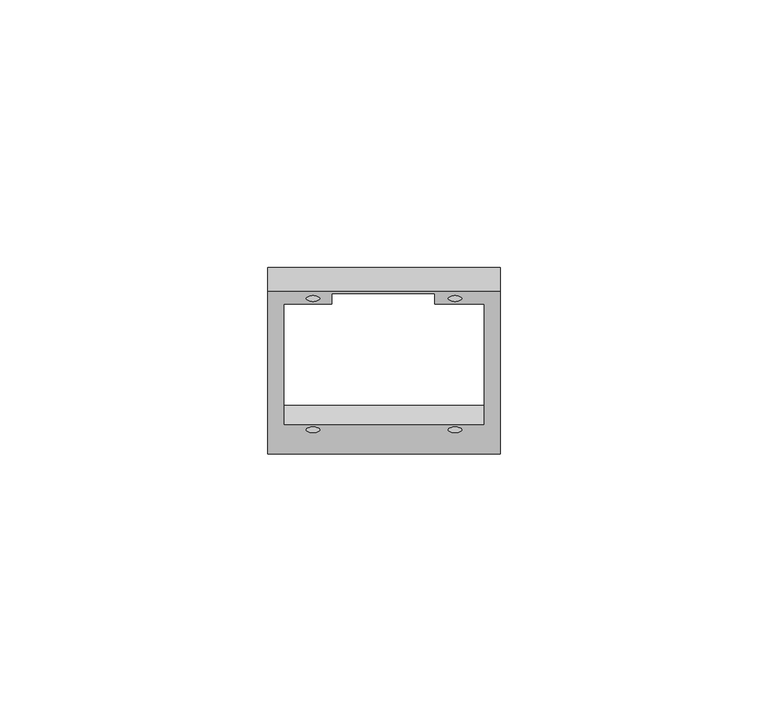
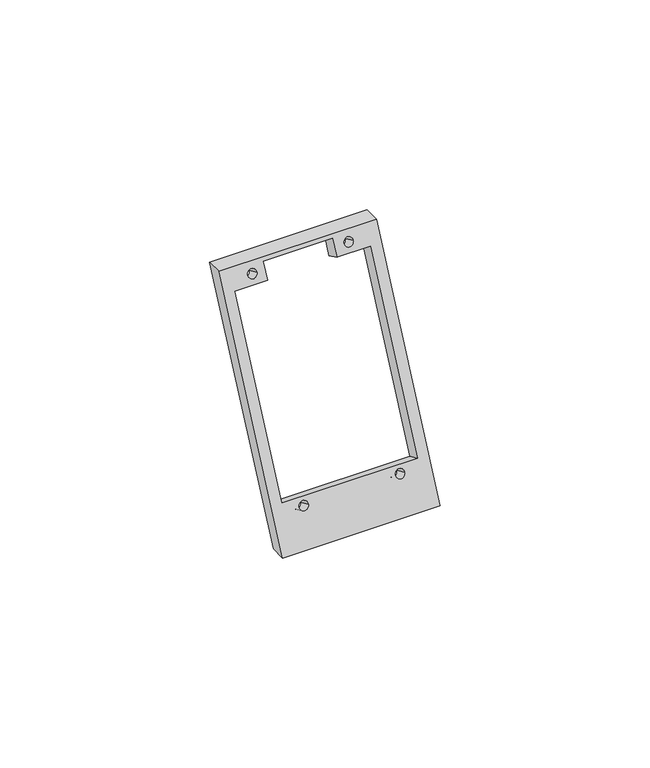
"""IFC4 building model written with IfcOpenShell, lengths in millimetres: furniture geometry, MOLDURA TELA : MOLDURA TELA."""

import ifcopenshell
import ifcopenshell.guid

model = None  # the IFC model being written
_history = None  # IfcOwnerHistory: only IFC2X3 demands one
_inside = {}  # id of a spatial element -> (the spatial element, [elements in it])
_under = {}  # id of a project, library or spatial element -> (it, [spatial elements below it])
_declared = {}  # id of a project -> (the project, [libraries it declares])
_typed = {}  # id of a type object -> (the type object, [elements of that type])
_made_of = {}  # id of a material, layer set ... -> (it, [elements and type objects made of it])


def new_model(schema):
    """Start an empty IFC model of exactly this schema.

    Asked for "IFC4X3", IfcOpenShell would pick the latest addendum, in which some entities
    have other attributes; the version numbers below select the first issue.
    IFC2X3 requires an IfcOwnerHistory on every rooted entity: one is made here for all.
    """
    global model, _history
    if schema == "IFC4X3":
        model = ifcopenshell.file(schema_version=(4, 3, 0, 0))
    else:
        model = ifcopenshell.file(schema=schema)
    _inside.clear()
    _under.clear()
    _declared.clear()
    _typed.clear()
    _made_of.clear()
    _history = None
    if model.schema == "IFC2X3":
        org = make("IfcOrganization", Name="unknown")
        user = make(
            "IfcPersonAndOrganization",
            ThePerson=make("IfcPerson", FamilyName="unknown"),
            TheOrganization=org,
        )
        app = make(
            "IfcApplication",
            ApplicationDeveloper=org,
            Version="unknown",
            ApplicationFullName="unknown",
            ApplicationIdentifier="unknown",
        )
        _history = make(
            "IfcOwnerHistory",
            OwningUser=user,
            OwningApplication=app,
            ChangeAction="ADDED",
            CreationDate=0,
        )
    return model


def make(cls, **values):
    """One entity of the class cls with the attributes given. An attribute that is None is left unset."""
    return model.create_entity(
        cls, **{name: value for name, value in values.items() if value is not None}
    )


def rooted(cls, **values):
    """An entity with a GlobalId (a new one), such as an element, a storey or a relation."""
    return make(cls, GlobalId=ifcopenshell.guid.new(), OwnerHistory=_history, **values)


def si_unit(unit_type, name, prefix=None):
    """IfcSIUnit, for example si_unit("LENGTHUNIT", "METRE", prefix="MILLI")."""
    return make("IfcSIUnit", UnitType=unit_type, Prefix=prefix, Name=name)


def assignment(units):
    """IfcUnitAssignment: the units of a project."""
    return None if units is None else make("IfcUnitAssignment", Units=units)


def point(xyz):
    """IfcCartesianPoint."""
    return None if xyz is None else make("IfcCartesianPoint", Coordinates=xyz)


def direction(xyz):
    """IfcDirection."""
    return None if xyz is None else make("IfcDirection", DirectionRatios=xyz)


def frame(location, z_axis=None, x_axis=None):
    """IfcAxis2Placement3D, a coordinate frame: its origin and axes. An axis left out is left unset."""
    return make(
        "IfcAxis2Placement3D",
        Location=point(location),
        Axis=direction(z_axis),
        RefDirection=direction(x_axis),
    )


def origin():
    """The frame at (0, 0, 0) with its axes left unset."""
    return frame((0.0, 0.0, 0.0))


def place(relative_to, where):
    """IfcLocalPlacement: puts the frame where relative to a parent placement (None: the world)."""
    return make(
        "IfcLocalPlacement", PlacementRelTo=relative_to, RelativePlacement=where
    )


def context(
    kind, dimensions, precision=None, world=None, true_north=None, identifier=None
):
    """IfcGeometricRepresentationContext, for example the 3D "Model" context."""
    return make(
        "IfcGeometricRepresentationContext",
        ContextIdentifier=identifier,
        ContextType=kind,
        CoordinateSpaceDimension=dimensions,
        Precision=precision,
        WorldCoordinateSystem=world,
        TrueNorth=true_north,
    )


def project(units=None, contexts=None):
    """IfcProject with its units and contexts."""
    return rooted(
        "IfcProject",
        Name="project",
        RepresentationContexts=contexts,
        UnitsInContext=assignment(units),
    )


def spatial(cls, under=None, at=None, **own):
    """A site, building, storey or space (cls), placed at a placement, below another one or the project."""
    s = rooted(cls, ObjectPlacement=at, **own)
    if under is not None:
        _under.setdefault(under.id(), (under, []))[1].append(s)
    return s


def polyline(points):
    """IfcPolyline through the points."""
    return make("IfcPolyline", Points=[point(p) for p in points])


def circle_curve(where, radius):
    """IfcCircle in the frame where."""
    return make("IfcCircle", Position=where, Radius=radius)


def shape(context_of_items, identifier, shape_type, items):
    """IfcShapeRepresentation: the items that make up one representation, for example the "Body"."""
    return make(
        "IfcShapeRepresentation",
        ContextOfItems=context_of_items,
        RepresentationIdentifier=identifier,
        RepresentationType=shape_type,
        Items=items,
    )


def source(mapping_origin, context_of_items, identifier, shape_type, items):
    """IfcRepresentationMap: a shape defined once, which mapped items show again and again."""
    return make(
        "IfcRepresentationMap",
        MappingOrigin=mapping_origin,
        MappedRepresentation=shape(context_of_items, identifier, shape_type, items),
    )


def transform(
    local_origin,
    x_axis=None,
    y_axis=None,
    z_axis=None,
    scale=None,
    scale2=None,
    scale3=None,
    uniform=True,
):
    """IfcCartesianTransformationOperator3D, or its non-uniform kind. x_axis, y_axis, z_axis: its Axis1, 2, 3."""
    if uniform:
        return make(
            "IfcCartesianTransformationOperator3D",
            Axis1=direction(x_axis),
            Axis2=direction(y_axis),
            LocalOrigin=point(local_origin),
            Scale=scale,
            Axis3=direction(z_axis),
        )
    return make(
        "IfcCartesianTransformationOperator3DnonUniform",
        Axis1=direction(x_axis),
        Axis2=direction(y_axis),
        LocalOrigin=point(local_origin),
        Scale=scale,
        Axis3=direction(z_axis),
        Scale2=scale2,
        Scale3=scale3,
    )


def mapped(mapping_source, mapping_target):
    """IfcMappedItem: shows the shape of a source again, moved by a transform."""
    return make(
        "IfcMappedItem", MappingSource=mapping_source, MappingTarget=mapping_target
    )


def made_of(thing, what):
    """Note that an element or type object is made of a material, layer set ...; save() writes the relation."""
    if what is not None:
        _made_of.setdefault(what.id(), (what, []))[1].append(thing)
    return thing


def element(
    cls,
    number,
    at=None,
    inside=None,
    cuts=None,
    type_object=None,
    material=None,
    context=None,
    identifier="Body",
    shape_type=None,
    held_by="IfcProductDefinitionShape",
    body=None,
    shapes=None,
    **own,
):
    """One element of the class cls, such as IfcWall. Its Tag is "e" and its number.

    at: its placement. inside: the storey or other place that contains it. cuts: it is an
    opening in that element (IfcRelVoidsElement). A single representation is given by context,
    identifier, shape_type and body (its items); several are given by shapes. held_by: the class
    of the entity that holds the representations. save() writes the other relations.
    """
    e = rooted(cls, Tag="e%d" % number, ObjectPlacement=at, **own)
    if body is not None:
        shapes = [shape(context, identifier, shape_type, body)]
    if shapes is not None:
        e.Representation = make(held_by, Representations=shapes)
    if inside is not None:
        _inside.setdefault(inside.id(), (inside, []))[1].append(e)
    if cuts is not None:
        rooted(
            "IfcRelVoidsElement", RelatingBuildingElement=cuts, RelatedOpeningElement=e
        )
    if type_object is not None:
        _typed.setdefault(type_object.id(), (type_object, []))[1].append(e)
    return made_of(e, material)


def aggregate(whole, parts):
    """IfcRelAggregates: a whole, such as a stair, and the parts it consists of."""
    return rooted("IfcRelAggregates", RelatingObject=whole, RelatedObjects=parts)


def save(model, path):
    """Write the relations noted so far, then the file.

    IfcRelAggregates (storeys below a building ...), IfcRelContainedInSpatialStructure (elements
    in a storey), IfcRelDefinesByType, IfcRelAssociatesMaterial and IfcRelDeclares: one each for
    every whole, place, type object, material and project.
    """
    for whole, parts in _under.values():
        aggregate(whole, parts)
    for where, things in _inside.values():
        rooted(
            "IfcRelContainedInSpatialStructure",
            RelatedElements=things,
            RelatingStructure=where,
        )
    for kind, things in _typed.values():
        rooted("IfcRelDefinesByType", RelatedObjects=things, RelatingType=kind)
    for what, things in _made_of.values():
        rooted("IfcRelAssociatesMaterial", RelatedObjects=things, RelatingMaterial=what)
    for by, libraries in _declared.values():
        rooted("IfcRelDeclares", RelatingContext=by, RelatedDefinitions=libraries)
    model.write(path)


def plane_surface(at):
    """IfcPlane: the flat surface through the origin of the frame at, square to its z axis."""
    return make("IfcPlane", Position=at)


def revolved_surface(curve, axis_point, axis_direction):
    """IfcSurfaceOfRevolution: the curve turned about the line through axis_point along axis_direction."""
    return make(
        "IfcSurfaceOfRevolution",
        SweptCurve=make("IfcArbitraryOpenProfileDef", ProfileType="CURVE", Curve=curve),
        AxisPosition=make("IfcAxis1Placement", Location=point(axis_point), Axis=direction(axis_direction)),
    )


def advanced_brep(points, edges, surfaces, faces):
    """IfcAdvancedBrep: a solid bounded by faces that lie on surfaces and meet in shared edges.

    An edge is (start, end): straight between two places in points (the first is 0);
    or (start, end, curve); or (start, end, curve, False) where it runs against its curve.
    A face is (place in surfaces, loops), or (place, loops, False) where it looks against
    its surface's normal. A loop lists edges by number (the first is 1), with a minus sign
    where the edge is run from its end to its start. The first loop is the outer one.
    """
    corners = [point(p) for p in points]
    vertices = [make("IfcVertexPoint", VertexGeometry=c) for c in corners]
    made = []
    for start, end, *more in edges:
        made.append(
            make(
                "IfcEdgeCurve",
                EdgeStart=vertices[start],
                EdgeEnd=vertices[end],
                EdgeGeometry=more[0] if more else make("IfcPolyline", Points=[corners[start], corners[end]]),
                SameSense=more[1] if len(more) > 1 else True,
            )
        )
    hull = []
    for where, loops, *sense in faces:
        bounds = []
        for j, loop in enumerate(loops):
            ring = [make("IfcOrientedEdge", EdgeElement=made[abs(k) - 1], Orientation=k > 0) for k in loop]
            bounds.append(
                make(
                    "IfcFaceOuterBound" if j == 0 else "IfcFaceBound",
                    Bound=make("IfcEdgeLoop", EdgeList=ring),
                    Orientation=True,
                )
            )
        hull.append(make("IfcAdvancedFace", Bounds=bounds, FaceSurface=surfaces[where], SameSense=sense[0] if sense else True))
    return make("IfcAdvancedBrep", Outer=make("IfcClosedShell", CfsFaces=hull))


def furniture_6c0b4a62(model_context):
    return source(origin(), model_context, "Body", "AdvancedBrep", [
        advanced_brep(
        [(2369.0719295, 1292.0509228, 0.0), (2369.0719295, 1322.3609206, 65.0), (2412.3719295, 1322.3609206, 65.0), (2412.3719295, 1292.0509228, 0.0), (2402.7219295, 1320.2478293, 60.4684611), (2405.2219295, 1320.2478293, 60.4684611), (2409.3719295, 1296.7079921, 9.9871173), (2409.3719295, 1319.10676, 58.02143), (2400.0719295, 1319.10676, 58.02143), (2400.0719295, 1321.0930658, 62.2810766), (2381.0719295, 1321.0930658, 62.2810766), (2381.0719295, 1319.10676, 58.02143), (2372.0719295, 1319.10676, 58.02143), (2372.0719295, 1296.7079921, 9.9871173), (2405.2219295, 1295.7359701, 7.9026094), (2402.7219295, 1295.7359701, 7.9026094), (2378.7219295, 1295.7359701, 7.9026094), (2376.2219295, 1295.7359701, 7.9026094), (2378.7219295, 1320.2478293, 60.4684611), (2376.2219295, 1320.2478293, 60.4684611), (2412.3719295, 1287.6374112, 0.0), (2412.3719295, 1317.9474089, 65.0), (2369.0719295, 1317.9474089, 65.0), (2369.0719295, 1287.6374112, 0.0), (2402.7219295, 1316.6225981, 62.1589341), (2405.2219295, 1316.6225981, 62.1589341), (2409.3719295, 1293.082761, 11.6775904), (2372.0719295, 1293.082761, 11.6775904), (2372.0719295, 1315.4815288, 59.7119031), (2381.0719295, 1315.4815288, 59.7119031), (2381.0719295, 1317.4678347, 63.9715497), (2400.0719295, 1317.4678347, 63.9715497), (2400.0719295, 1315.4815288, 59.7119031), (2409.3719295, 1315.4815288, 59.7119031), (2405.2219295, 1292.110739, 9.5930825), (2402.7219295, 1292.110739, 9.5930825), (2378.7219295, 1292.110739, 9.5930825), (2376.2219295, 1292.110739, 9.5930825), (2378.7219295, 1316.6225981, 62.1589341), (2376.2219295, 1316.6225981, 62.1589341)],
        [
            (0, 1),
            (1, 2),
            (2, 3),
            (3, 0),
            (4, 5, circle_curve(frame((2403.9719295, 1320.2478293, 60.4684611), z_axis=(0.0, -0.9063077870366535, 0.4226182617406919), x_axis=(-1.0, 0.0, 0.0)), 1.25)),
            (5, 4, circle_curve(frame((2403.9719295, 1320.2478293, 60.4684611), z_axis=(0.0, -0.9063077870366535, 0.4226182617406919), x_axis=(-1.0, 0.0, 0.0)), 1.25)),
            (6, 7),
            (7, 8),
            (8, 9),
            (9, 10),
            (10, 11),
            (11, 12),
            (12, 13),
            (13, 6),
            (14, 15, circle_curve(frame((2403.9719295, 1295.7359701, 7.9026094), z_axis=(0.0, -0.9063077870366535, 0.4226182617406919), x_axis=(-1.0, 0.0, 0.0)), 1.25)),
            (15, 14, circle_curve(frame((2403.9719295, 1295.7359701, 7.9026094), z_axis=(0.0, -0.9063077870366535, 0.4226182617406919), x_axis=(-1.0, 0.0, 0.0)), 1.25)),
            (16, 17, circle_curve(frame((2377.4719295, 1295.7359701, 7.9026094), z_axis=(0.0, -0.9063077870366535, 0.4226182617406919), x_axis=(1.0, 0.0, 0.0)), 1.25)),
            (17, 16, circle_curve(frame((2377.4719295, 1295.7359701, 7.9026094), z_axis=(0.0, -0.9063077870366535, 0.4226182617406919), x_axis=(1.0, 0.0, 0.0)), 1.25)),
            (18, 19, circle_curve(frame((2377.4719295, 1320.2478293, 60.4684611), z_axis=(0.0, -0.9063077870366535, 0.4226182617406919), x_axis=(1.0, 0.0, 0.0)), 1.25)),
            (19, 18, circle_curve(frame((2377.4719295, 1320.2478293, 60.4684611), z_axis=(0.0, -0.9063077870366535, 0.4226182617406919), x_axis=(1.0, 0.0, 0.0)), 1.25)),
            (20, 21),
            (21, 22),
            (22, 23),
            (23, 20),
            (24, 25, circle_curve(frame((2403.9719295, 1316.6225981, 62.1589341), z_axis=(0.0, 0.9063077870366535, -0.4226182617406919), x_axis=(-1.0, 0.0, 0.0)), 1.25)),
            (25, 24, circle_curve(frame((2403.9719295, 1316.6225981, 62.1589341), z_axis=(0.0, 0.9063077870366535, -0.4226182617406919), x_axis=(-1.0, 0.0, 0.0)), 1.25)),
            (26, 27),
            (27, 28),
            (28, 29),
            (29, 30),
            (30, 31),
            (31, 32),
            (32, 33),
            (33, 26),
            (34, 35, circle_curve(frame((2403.9719295, 1292.110739, 9.5930825), z_axis=(0.0, 0.9063077870366535, -0.4226182617406919), x_axis=(-1.0, 0.0, 0.0)), 1.25)),
            (35, 34, circle_curve(frame((2403.9719295, 1292.110739, 9.5930825), z_axis=(0.0, 0.9063077870366535, -0.4226182617406919), x_axis=(-1.0, 0.0, 0.0)), 1.25)),
            (36, 37, circle_curve(frame((2377.4719295, 1292.110739, 9.5930825), z_axis=(0.0, 0.9063077870366535, -0.4226182617406919), x_axis=(1.0, 0.0, 0.0)), 1.25)),
            (37, 36, circle_curve(frame((2377.4719295, 1292.110739, 9.5930825), z_axis=(0.0, 0.9063077870366535, -0.4226182617406919), x_axis=(1.0, 0.0, 0.0)), 1.25)),
            (38, 39, circle_curve(frame((2377.4719295, 1316.6225981, 62.1589341), z_axis=(0.0, 0.9063077870366535, -0.4226182617406919), x_axis=(1.0, 0.0, 0.0)), 1.25)),
            (39, 38, circle_curve(frame((2377.4719295, 1316.6225981, 62.1589341), z_axis=(0.0, 0.9063077870366535, -0.4226182617406919), x_axis=(1.0, 0.0, 0.0)), 1.25)),
            (0, 23),
            (22, 1),
            (2, 21),
            (20, 3),
            (4, 24),
            (25, 5),
            (6, 26),
            (33, 7),
            (32, 8),
            (31, 9),
            (30, 10),
            (29, 11),
            (28, 12),
            (27, 13),
            (14, 34),
            (35, 15),
            (16, 36),
            (37, 17),
            (18, 38),
            (39, 19),
        ],
        [
            plane_surface(frame((2369.0719295, 1293.6228788, 3.3710705), z_axis=(0.0, 0.9063077870366535, -0.4226182617406919), x_axis=(0.0, 0.4226182617406919, 0.9063077870366535))),
            plane_surface(frame((2369.0719295, 1289.9976477, 5.0615435), z_axis=(0.0, -0.9063077870366535, 0.4226182617406919), x_axis=(0.0, -0.4226182617406919, -0.9063077870366535))),
            plane_surface(frame((2369.0719295, 1290.6199639, -3.0687014), z_axis=(-1.0, 0.0, 0.0), x_axis=(0.0, -0.9063077870366527, 0.42261826174069356))),
            plane_surface(frame((2412.3719295, 1322.3609206, 65.0), z_axis=(1.0, 0.0, 0.0), x_axis=(0.0, -0.9063077870366535, 0.42261826174069184))),
            revolved_surface(polyline([(2402.7219295, 1316.6225981272491, 62.15893415843589), (2402.7219295, 1320.2478293, 60.4684611)]), (2403.9719295, 1320.2478293, 60.4684611), (0.0, -0.9063077870366535, 0.4226182617406919)),
            plane_surface(frame((2409.3719295, 1296.7079921, 9.9871173), z_axis=(-1.0, 0.0, 0.0), x_axis=(0.0, -0.9063077870366532, 0.4226182617406927))),
            plane_surface(frame((2409.3719295, 1319.10676, 58.02143), z_axis=(0.0, -0.42261826174069184, -0.9063077870366535), x_axis=(0.0, -0.9063077870366535, 0.42261826174069184))),
            plane_surface(frame((2400.0719295, 1319.10676, 58.02143), z_axis=(-1.0, 0.0, 0.0), x_axis=(0.0, -0.9063077870366535, 0.42261826174069184))),
            plane_surface(frame((2400.0719295, 1321.0930658, 62.2810766), z_axis=(0.0, -0.42261826174069184, -0.9063077870366535), x_axis=(0.0, -0.9063077870366535, 0.42261826174069184))),
            plane_surface(frame((2381.0719295, 1321.0930658, 62.2810766), z_axis=(1.0, 0.0, 0.0), x_axis=(0.0, -0.9063077870366527, 0.42261826174069356))),
            plane_surface(frame((2381.0719295, 1319.10676, 58.02143), z_axis=(0.0, -0.42261826174069184, -0.9063077870366535), x_axis=(0.0, -0.9063077870366535, 0.42261826174069184))),
            plane_surface(frame((2372.0719295, 1319.10676, 58.02143), z_axis=(1.0, 0.0, 0.0), x_axis=(0.0, -0.9063077870366535, 0.42261826174069184))),
            plane_surface(frame((2372.0719295, 1296.7079921, 9.9871173), z_axis=(0.0, 0.4226182617406927, 0.9063077870366532), x_axis=(0.0, -0.9063077870366532, 0.4226182617406927))),
            revolved_surface(polyline([(2402.7219295, 1292.1107389710862, 9.593082437994347), (2402.7219295, 1295.7359701, 7.9026094)]), (2403.9719295, 1295.7359701, 7.9026094), (0.0, -0.9063077870366535, 0.4226182617406919)),
            revolved_surface(polyline([(2378.7219295, 1292.1107389710862, 9.593082437994347), (2378.7219295, 1295.7359701, 7.9026094)]), (2377.4719295, 1295.7359701, 7.9026094), (0.0, -0.9063077870366535, 0.4226182617406919)),
            revolved_surface(polyline([(2378.7219295, 1316.6225981272491, 62.15893415843589), (2378.7219295, 1320.2478293, 60.4684611)]), (2377.4719295, 1320.2478293, 60.4684611), (0.0, -0.9063077870366535, 0.4226182617406919)),
            plane_surface(frame((2418.7000554, 1312.6608189, 65.0), z_axis=(0.0, 0.0, 1.0), x_axis=(-1.0, 0.0, 0.0))),
            plane_surface(frame((2418.7000554, 1302.9468274, 0.0), z_axis=(0.0, 0.0, -1.0), x_axis=(-1.0, 0.0, 0.0))),
        ],
        [
            (0, [[1, 2, 3, 4], [5, 6], [7, 8, 9, 10, 11, 12, 13, 14], [15, 16], [17, 18], [19, 20]]),
            (1, [[21, 22, 23, 24], [25, 26], [27, 28, 29, 30, 31, 32, 33, 34], [35, 36], [37, 38], [39, 40]]),
            (2, [[-1, 41, -23, 42]]),
            (3, [[-3, 43, -21, 44]]),
            (4, [[-5, 45, -26, 46]]),
            (4, [[-6, -46, -25, -45]]),
            (5, [[-7, 47, -34, 48]]),
            (6, [[-8, -48, -33, 49]]),
            (7, [[-9, -49, -32, 50]]),
            (8, [[-10, -50, -31, 51]]),
            (9, [[-11, -51, -30, 52]]),
            (10, [[-12, -52, -29, 53]]),
            (11, [[-13, -53, -28, 54]]),
            (12, [[-14, -54, -27, -47]]),
            (13, [[-15, 55, -36, 56]]),
            (13, [[-16, -56, -35, -55]]),
            (14, [[-17, 57, -38, 58]]),
            (14, [[-18, -58, -37, -57]]),
            (15, [[-19, 59, -40, 60]]),
            (15, [[-20, -60, -39, -59]]),
            (16, [[-2, -42, -22, -43]]),
            (17, [[-4, -44, -24, -41]]),
        ],
    ),
    ])


if __name__ == "__main__":
    model = new_model("IFC4")
    model_context = context("Model", 3, world=origin())
    ifc_project = project(units=[si_unit("LENGTHUNIT", "METRE", prefix="MILLI")], contexts=[model_context])
    site = spatial("IfcSite", under=ifc_project)
    building = spatial("IfcBuilding", under=site)
    placement = place(None, origin())
    furniture_shape = furniture_6c0b4a62(model_context)
    element("IfcFurniture", 1, ObjectType="MOLDURA TELA : MOLDURA TELA", at=placement, inside=building, context=model_context, shape_type="MappedRepresentation", body=[
        mapped(furniture_shape, transform((0.0, 0.0, 0.0), x_axis=(1.0, 0.0, 0.0), y_axis=(0.0, 1.0, 0.0), z_axis=(0.0, 0.0, 1.0))),
    ])
    save(model, "model.ifc")

# Revit data of these elements
# Project information
#   Data de emissão do projeto = "Data de emissão"
#   Status do projeto = "Status do projeto"
#   Nome do cliente = "Proprietário"
#   Endereço do projeto = "Insira aqui o endereço"
#   Nome do projeto = "Nome do projeto"
#   Número do projeto = "0001"
# Type "MOLDURA TELA : MOLDURA TELA"
#   Height = 0
# Element 1 (IfcFurniture, "MOLDURA TELA : MOLDURA TELA")
#   Materials on its faces: ".BOX FUNDO"
# Materials
#   ".BOX FUNDO": class "Vidro", colour RGB 236 240 239, transparency 0.15, Cost = 0
